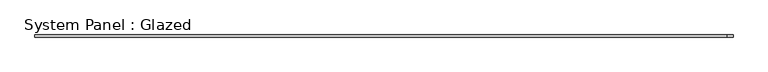
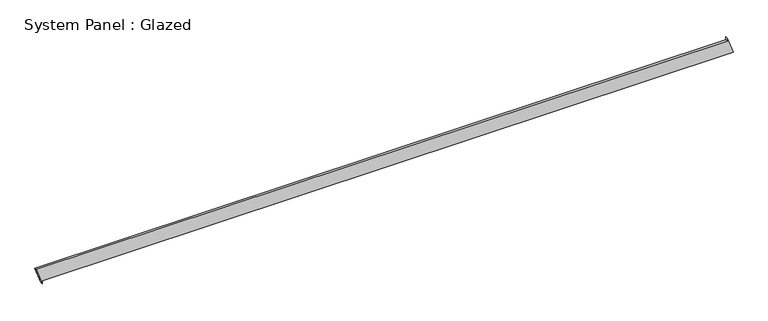
"""IFC4 building model written with IfcOpenShell, lengths in millimetres: plate geometry, System Panel : Glazed."""

from ifc_helpers import new_model, si_unit, frame, origin, place, context, project, spatial, polyline, outline, extrude, source, transform, mapped, element, save


def system_panel_glazed_1248680a(model_context):
    return source(origin(), model_context, "Body", "SweptSolid", [
        extrude(outline(polyline([(0.0, -3958.7701168), (35.3553391, -3958.7701168), (35.3553391, 4027.9908618), (234.4800551, 3958.6624486), (199.124716, 3958.6622495), (199.1697072, -4027.9908618), (0.0, -3958.7701168)])), frame((0.0, -49.5, 0.0), z_axis=(0.0, 1.0, 0.0), x_axis=(0.0, 0.0, 1.0)), (0.0, 0.0, 1.0), 25.0),
    ])


if __name__ == "__main__":
    model = new_model("IFC4")
    model_context = context("Model", 3, world=origin())
    ifc_project = project(units=[si_unit("LENGTHUNIT", "METRE", prefix="MILLI")], contexts=[model_context])
    site = spatial("IfcSite", under=ifc_project)
    building = spatial("IfcBuilding", under=site)
    placement = place(None, origin())
    system_panel_glazed_shape = system_panel_glazed_1248680a(model_context)
    element("IfcPlate", 1, ObjectType="System Panel : Glazed", at=placement, inside=building, context=model_context, shape_type="MappedRepresentation", body=[
        mapped(system_panel_glazed_shape, transform((0.0, 0.0, 0.0), x_axis=(1.0, 0.0, 0.0), y_axis=(0.0, 1.0, 0.0), z_axis=(0.0, 0.0, 1.0))),
    ])
    save(model, "model.ifc")

# Revit data of these elements
# Element 1 (IfcPlate, "System Panel : Glazed")
#   Materials on its faces: "Glass"
# Materials
#   "Glass": class "Glass", colour RGB 218 227 224, transparency 0.85, Description = "Soda Lime Glass", Cost = 0
